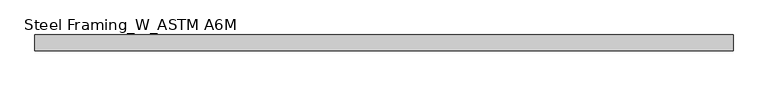
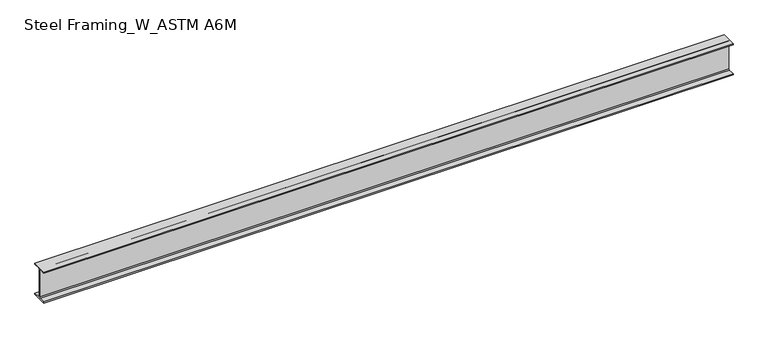
"""IFC4 building model written with IfcOpenShell, lengths in millimetres: beam geometry, Steel Framing_W_ASTM A6M : H_SB_AR_S02_W360x51_RG1."""

from ifc_helpers import new_model, si_unit, point, frame, frame_2d, origin, place, context, project, spatial, polyline, circle_curve, trimmed, segment, composite_curve, outline, extrude, source, transform, mapped, element, save


def steel_framing_w_astm_a6m_b27ce7d5(model_context):
    return source(origin(), model_context, "Body", "SweptSolid", [
        extrude(outline(composite_curve([segment(polyline([(85.5, -166.4), (85.5, -178.0), (-85.5, -178.0), (-85.5, -166.4), (-13.72, -166.4)]), True, "CONTINUOUS"), segment(trimmed(circle_curve(frame_2d((-13.72, -156.3)), 10.1), [point((-13.72, -166.4))], [point((-3.62, -156.3))], True, "CARTESIAN"), True, "CONTINUOUS"), segment(polyline([(-3.62, -156.3), (-3.62, 156.3)]), True, "CONTINUOUS"), segment(trimmed(circle_curve(frame_2d((-13.72, 156.3)), 10.1), [point((-3.62, 156.3))], [point((-13.72, 166.4))], True, "CARTESIAN"), True, "CONTINUOUS"), segment(polyline([(-13.72, 166.4), (-85.5, 166.4), (-85.5, 178.0), (85.5, 178.0), (85.5, 166.4), (13.72, 166.4)]), True, "CONTINUOUS"), segment(trimmed(circle_curve(frame_2d((13.72, 156.3)), 10.1), [point((13.72, 166.4))], [point((3.62, 156.3))], True, "CARTESIAN"), True, "CONTINUOUS"), segment(polyline([(3.62, 156.3), (3.62, -156.3)]), True, "CONTINUOUS"), segment(trimmed(circle_curve(frame_2d((13.72, -156.3)), 10.1), [point((3.62, -156.3))], [point((13.72, -166.4))], True, "CARTESIAN"), True, "CONTINUOUS"), segment(polyline([(13.72, -166.4), (85.5, -166.4)]), True, "CONTINUOUS")], self_intersect=False)), frame((-3736.95, 0.0, 0.0), z_axis=(1.0, 0.0, 0.0), x_axis=(0.0, 1.0, 0.0)), (0.0, 0.0, 1.0), 7511.8),
    ])


if __name__ == "__main__":
    model = new_model("IFC4")
    model_context = context("Model", 3, world=origin())
    ifc_project = project(units=[si_unit("LENGTHUNIT", "METRE", prefix="MILLI")], contexts=[model_context])
    site = spatial("IfcSite", under=ifc_project)
    building = spatial("IfcBuilding", under=site)
    placement = place(None, origin())
    steel_framing_w_astm_a6m_shape = steel_framing_w_astm_a6m_b27ce7d5(model_context)
    element("IfcBeam", 1, ObjectType="Steel Framing_W_ASTM A6M : H_SB_AR_S02_W360x51_RG1", at=placement, inside=building, context=model_context, shape_type="MappedRepresentation", body=[
        mapped(steel_framing_w_astm_a6m_shape, transform((0.0, 0.0, 0.0), x_axis=(1.0, 0.0, 0.0), y_axis=(0.0, 1.0, 0.0), z_axis=(0.0, 0.0, 1.0))),
    ])
    save(model, "model.ifc")

# Revit data of these elements
# Type "Steel Framing_W_ASTM A6M : H_SB_AR_S02_W360x51_RG1"
#   Section Name Key = "W14x34"
#   Width = 17.1 cm
#   Web Thickness = 0.724 cm
#   Web Fillet = 1.01 cm
#   Warping Constant = 287000.0 cm⁶
#   Torsional Moment of Inertia = 23.70 cm⁴
#   Section Area = 64.5 cm²
#   Plastic Modulus weak axis = 174.0 cm³
#   Plastic Modulus strong axis = 895.0 cm³
#   Perimeter = 1.36 m²/m
#   Nominal Weight = 51.00 kgf/m
#   Moment of Inertia weak axis = 970.00 cm⁴
#   Moment of Inertia strong axis = 14200.00 cm⁴
#   Height = 35.6 cm
#   Flange Thickness = 1.16 cm
#   Elastic Modulus weak axis = 113.0 cm³
#   Elastic Modulus strong axis = 796.0 cm³
#   Centroid Vertical = 17.8 cm
#   Centroid Horizontal = 8.55 cm
#   Length [instance default] = 1500 mm
#   Structural Material [instance default] = Steel, 45-345
#   Bolt Spacing = 0
#   Assembly Code = ""
# Element 1 (IfcBeam, "Steel Framing_W_ASTM A6M : H_SB_AR_S02_W360x51_RG1")
#   Materials on its faces: "Steel, 45-345"
# Materials
#   "Steel, 45-345": class "Metal", colour RGB 189 187 185, transparency 0, Description = "Steel 345 MPa", Cost = 0
